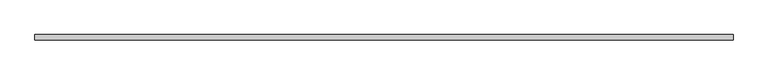
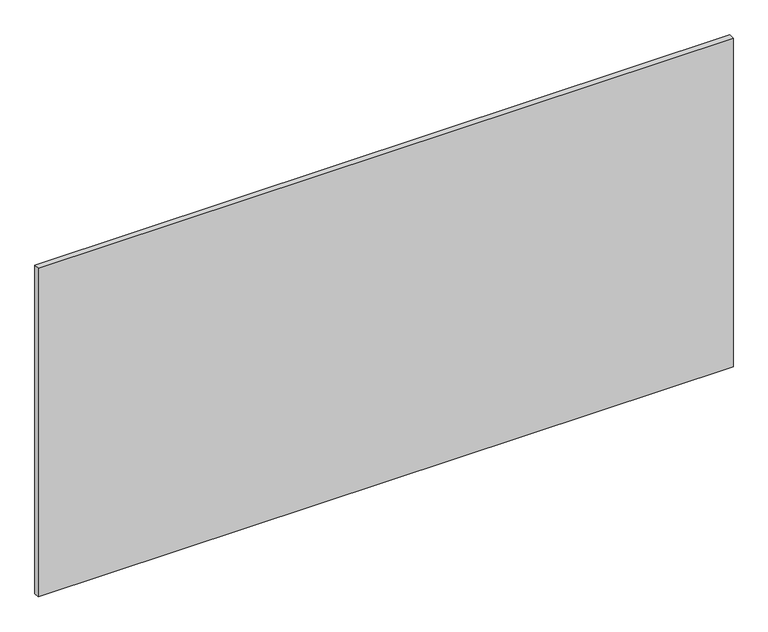
"""IFC4 building model written with IfcOpenShell, lengths in millimetres: proxy geometry, Inner panel:Inner panel:1:Inner panel:1 : Inner panel:Inner panel:300324:300043:Inner panel:1:Inner panel:1 : Inner panel:Inner panel:300324:300043 : Inner panel:Inner panel:1:Inner panel:1 : Inner panel:Inner panel:300324:300043:17 : Inner panel:Inner panel:1:Inner panel:1 : Inner panel:Inner panel:300324:300043:Inner panel:1:Inner panel:1 : Inner panel:Inner panel:300324:300043 : Inner panel:Inner panel:1:Inner panel:1 : Inner panel:Inner panel:300324:300043:300031."""

from ifc_helpers import new_model, si_unit, frame, origin, place, context, project, spatial, polyline, outline, extrude, source, transform, mapped, element, save


def generic_models_5892a33f(model_context):
    return source(origin(), model_context, "Body", "SweptSolid", [
        extrude(outline(polyline([(593738.0867239, -568186.6413841), (596176.4867239, -568186.6413841), (596176.4867239, -568205.6913841), (593738.0867239, -568205.6913841), (593738.0867239, -568186.6413841)])), frame((0.0, 0.0, 2495.55), z_axis=(0.0, 0.0, 1.0), x_axis=(1.0, 0.0, 0.0)), (0.0, 0.0, 1.0), 1219.2),
    ])


if __name__ == "__main__":
    model = new_model("IFC4")
    model_context = context("Model", 3, world=origin())
    ifc_project = project(units=[si_unit("LENGTHUNIT", "METRE", prefix="MILLI")], contexts=[model_context])
    site = spatial("IfcSite", under=ifc_project)
    building = spatial("IfcBuilding", under=site)
    placement = place(None, origin())
    generic_models_shape = generic_models_5892a33f(model_context)
    element("IfcBuildingElementProxy", 1, Name="Inner panel:Inner panel:1:Inner panel:1 : Inner panel:Inner panel:300324:300043:Inner panel:1:Inner panel:1 : Inner panel:Inner panel:300324:300043 : Inner panel:Inner panel:1:Inner panel:1 : Inner panel:Inner panel:300324:300043:17 : Inner panel:Inner panel:1:Inner panel:1 : Inner panel:Inner panel:300324:300043:Inner panel:1:Inner panel:1 : Inner panel:Inner panel:300324:300043 : Inner panel:Inner panel:1:Inner panel:1 : Inner panel:Inner panel:300324:300043:300031", ObjectType="Inner panel:Inner panel:1:Inner panel:1 : Inner panel:Inner panel:300324:300043:Inner panel:1:Inner panel:1 : Inner panel:Inner panel:300324:300043 : Inner panel:Inner panel:1:Inner panel:1 : Inner panel:Inner panel:300324:300043:17 : Inner panel:Inner panel:1:Inner panel:1 : Inner panel:Inner panel:300324:300043:Inner panel:1:Inner panel:1 : Inner panel:Inner panel:300324:300043 : Inner panel:Inner panel:1:Inner panel:1 : Inner panel:Inner panel:300324:300043:300031", at=placement, inside=building, context=model_context, shape_type="MappedRepresentation", body=[
        mapped(generic_models_shape, transform((0.0, 0.0, 0.0), x_axis=(1.0, 0.0, 0.0), y_axis=(0.0, 1.0, 0.0), z_axis=(0.0, 0.0, 1.0))),
    ])
    save(model, "model.ifc")

# Revit data of these elements
# Type "Inner panel:Inner panel:1:Inner panel:1 : Inner panel:Inner panel:300324:300043:Inner panel:1:Inner panel:1 : Inner panel:Inner panel:300324:300043 : Inner panel:Inner panel:1:Inner panel:1 : Inner panel:Inner panel:300324:300043:17 : Inner panel:Inner panel:1:Inner panel:1 : Inner panel:Inner panel:300324:300043:Inner panel:1:Inner panel:1 : Inner panel:Inner panel:300324:300043 : Inner panel:Inner panel:1:Inner panel:1 : Inner panel:Inner panel:300324:300043:300031"
#   NameOverride = "Inner panel:Inner panel:1:Inner panel:1 : Inner panel:Inner panel:300324:300043:Inner panel:1:Inner panel:1 : Inner panel:Inner panel:300324:300043 : Inner panel:Inner panel:1:Inner panel:1 : Inner panel:Inner panel:300324:300043:300031"
#   ObjectTypeOverride = "Inner panel:1:Inner panel:1 : Inner panel:Inner panel:300324:300043 : Inner panel:Inner panel:1:Inner panel:1 : Inner panel:Inner panel:300324:300043"
#   Reference = "Inner panel"
#   Tag = "300031"
# Element 1 (IfcBuildingElementProxy, "Inner panel:Inner panel:1:Inner panel:1 : Inner panel:Inner panel:300324:300043:Inner panel:1:Inner panel:1 : Inner panel:Inner panel:300324:300043 : Inner panel:Inner panel:1:Inner panel:1 : Inner panel:Inner panel:300324:300043:17 : Inner panel:Inner panel:1:Inner panel:1 : Inner panel:Inner panel:300324:300043:Inner panel:1:Inner panel:1 : Inner panel:Inner panel:300324:300043 : Inner panel:Inner panel:1:Inner panel:1 : Inner panel:Inner panel:300324:300043:300031")
#   Materials on its faces: "¾” (CLASS A) FIRE RETARDANT PLYWOOD ...OR… IF 1/4\" GYP. BD UNDER PLYWOOD, FLAME SPREAD TO BE CLASS C -  (FINISH: GRADE B - PREFINISHED STAINED/SEALED) - 1/4\" GAP BTWN PANELS (FASTENERS T.B.D.)"
# Materials
#   "¾” (CLASS A) FIRE RETARDANT PLYWOOD ...OR… IF 1/4\" GYP. BD UNDER PLYWOOD, FLAME SPREAD TO BE CLASS C -  (FINISH: GRADE B - PREFINISHED STAINED/SEALED) - 1/4\" GAP BTWN PANELS (FASTENERS T.B.D.)": class "Wood", colour RGB 149 120 74, transparency 0, Description = "Plywood, sheathing grade", Cost = 0
